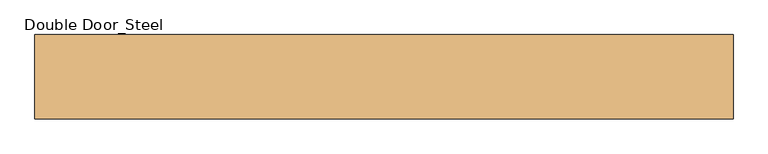
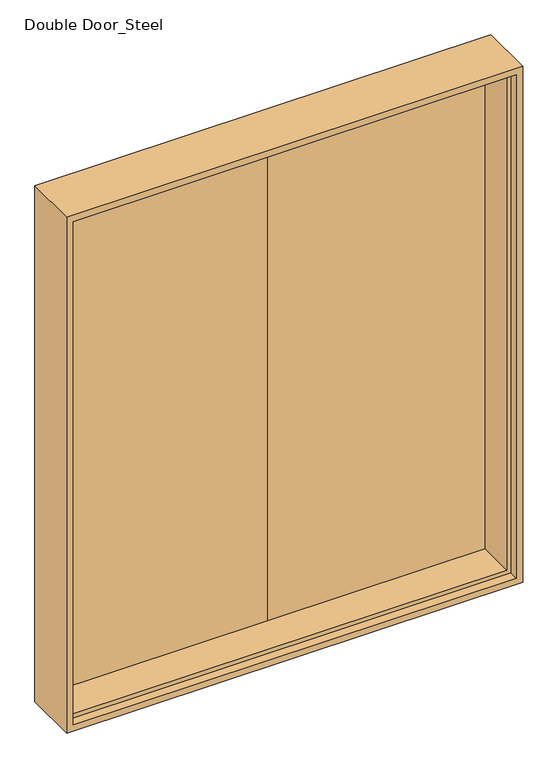
"""IFC4 building model written with IfcOpenShell, lengths in millimetres: door geometry, Double Door_Steel : H_DR_AR B12_Door_Double_W2100xH2490_FR 1.0H_FSD-3."""

from ifc_helpers import new_model, si_unit, frame, origin, place, context, project, spatial, polyline, outline, extrude, faceted_brep, source, transform, mapped, element, save


def double_door_steel_4b1f7132(model_context):
    return source(origin(), model_context, "Body", "SolidModel", [
        faceted_brep([(1035.0, -125.0, 2475.0), (1035.0, 125.0, 2475.0), (-1035.0, 125.0, 2475.0), (-1035.0, -125.0, 2475.0), (985.0, 85.0, 2425.0), (985.0, -85.0, 2425.0), (-985.0, -85.0, 2425.0), (-985.0, 85.0, 2425.0), (1005.0, 125.0, 2445.0), (1005.0, 85.0, 2445.0), (-1005.0, 85.0, 2445.0), (-1005.0, 125.0, 2445.0), (-1035.0, 125.0, 0.0), (-1035.0, -125.0, 0.0), (-985.0, -85.0, 50.0), (-985.0, 85.0, 50.0), (-1005.0, 85.0, 30.0), (-1005.0, 125.0, 30.0), (1035.0, 125.0, 0.0), (1005.0, 125.0, 30.0), (1035.0, -125.0, 0.0), (1005.0, -125.0, 30.0), (-1005.0, -125.0, 30.0), (-1005.0, -125.0, 2445.0), (1005.0, -125.0, 2445.0), (985.0, -85.0, 50.0), (985.0, 85.0, 50.0), (1005.0, 85.0, 30.0), (1005.0, -85.0, 30.0), (1005.0, -85.0, 2445.0), (-1005.0, -85.0, 2445.0), (-1005.0, -85.0, 30.0)], [[[0, 1, 2, 3]], [[4, 5, 6, 7]], [[8, 9, 10, 11]], [[3, 2, 12, 13]], [[7, 6, 14, 15]], [[11, 10, 16, 17]], [[18, 12, 2, 1], [8, 11, 17, 19]], [[13, 12, 18, 20]], [[0, 3, 13, 20], [21, 22, 23, 24]], [[15, 14, 25, 26]], [[27, 16, 10, 9], [4, 7, 15, 26]], [[17, 16, 27, 19]], [[20, 18, 1, 0]], [[26, 25, 5, 4]], [[19, 27, 9, 8]], [[28, 21, 24, 29]], [[29, 24, 23, 30]], [[30, 23, 22, 31]], [[30, 31, 28, 29], [5, 25, 14, 6]], [[31, 22, 21, 28]]]),
        extrude(outline(polyline([(1005.0, 85.0), (0.0, 85.0), (0.0, 125.0), (1005.0, 125.0), (1005.0, 85.0)])), frame((0.0, 0.0, 30.0), z_axis=(0.0, 0.0, 1.0), x_axis=(1.0, 0.0, 0.0)), (0.0, 0.0, 1.0), 2415.0),
        extrude(outline(polyline([(0.0, 85.0), (-1005.0, 85.0), (-1005.0, 125.0), (0.0, 125.0), (0.0, 85.0)])), frame((0.0, 0.0, 30.0), z_axis=(0.0, 0.0, 1.0), x_axis=(1.0, 0.0, 0.0)), (0.0, 0.0, 1.0), 2415.0),
    ])


if __name__ == "__main__":
    model = new_model("IFC4")
    model_context = context("Model", 3, world=origin())
    ifc_project = project(units=[si_unit("LENGTHUNIT", "METRE", prefix="MILLI")], contexts=[model_context])
    site = spatial("IfcSite", under=ifc_project)
    building = spatial("IfcBuilding", under=site)
    placement = place(None, origin())
    double_door_steel_shape = double_door_steel_4b1f7132(model_context)
    element("IfcDoor", 1, ObjectType="Double Door_Steel : H_DR_AR B12_Door_Double_W2100xH2490_FR 1.0H_FSD-3", at=placement, inside=building, context=model_context, shape_type="MappedRepresentation", body=[
        mapped(double_door_steel_shape, transform((0.0, 0.0, 0.0), x_axis=(1.0, 0.0, 0.0), y_axis=(0.0, 1.0, 0.0), z_axis=(0.0, 0.0, 1.0))),
    ])
    save(model, "model.ifc")

# Revit data of these elements
# Type "Double Door_Steel : H_DR_AR B12_Door_Double_W2100xH2490_FR 1.0H_FSD-3"
#   Type Mark = "443"
#   프레임 = ""
#   철물 = ""
#   유리/마감 = ""
#   위치/개소 = ""
#   부호 = ""
#   문번호 = ""
#   문기호 = "FSD-3"
#   Analytic Construction = "<None>"
#   Door Width = 1005 mm
#   Height = 2490 mm
#   Width = 2100 mm
#   Define Thermal Properties by = 1
#   문 틀 = none
#   문 = none
#   Function = (empty or 0)
#   Assembly Code = ""
#   Wall Closure = (empty or 0)
